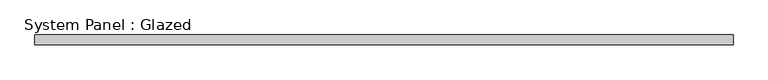
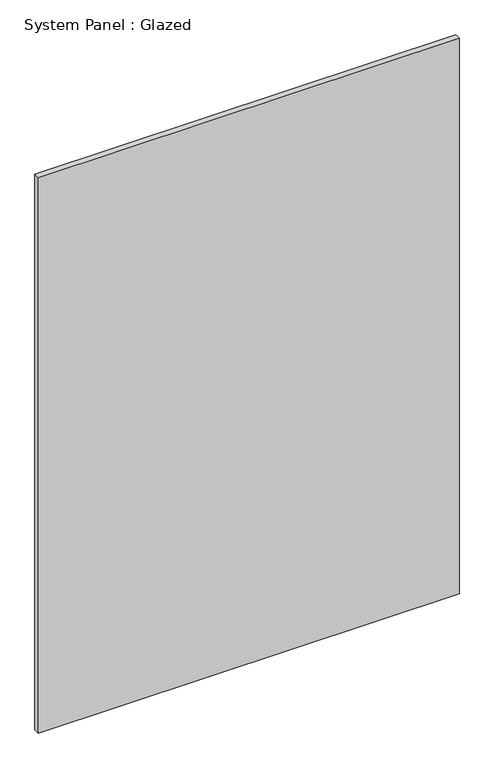
"""IFC4 building model written with IfcOpenShell, lengths in millimetres: plate geometry, System Panel : Glazed."""

import ifcopenshell
import ifcopenshell.guid

model = None  # the IFC model being written
_history = None  # IfcOwnerHistory: only IFC2X3 demands one
_inside = {}  # id of a spatial element -> (the spatial element, [elements in it])
_under = {}  # id of a project, library or spatial element -> (it, [spatial elements below it])
_declared = {}  # id of a project -> (the project, [libraries it declares])
_typed = {}  # id of a type object -> (the type object, [elements of that type])
_made_of = {}  # id of a material, layer set ... -> (it, [elements and type objects made of it])


def new_model(schema):
    """Start an empty IFC model of exactly this schema.

    Asked for "IFC4X3", IfcOpenShell would pick the latest addendum, in which some entities
    have other attributes; the version numbers below select the first issue.
    IFC2X3 requires an IfcOwnerHistory on every rooted entity: one is made here for all.
    """
    global model, _history
    if schema == "IFC4X3":
        model = ifcopenshell.file(schema_version=(4, 3, 0, 0))
    else:
        model = ifcopenshell.file(schema=schema)
    _inside.clear()
    _under.clear()
    _declared.clear()
    _typed.clear()
    _made_of.clear()
    _history = None
    if model.schema == "IFC2X3":
        org = make("IfcOrganization", Name="unknown")
        user = make(
            "IfcPersonAndOrganization",
            ThePerson=make("IfcPerson", FamilyName="unknown"),
            TheOrganization=org,
        )
        app = make(
            "IfcApplication",
            ApplicationDeveloper=org,
            Version="unknown",
            ApplicationFullName="unknown",
            ApplicationIdentifier="unknown",
        )
        _history = make(
            "IfcOwnerHistory",
            OwningUser=user,
            OwningApplication=app,
            ChangeAction="ADDED",
            CreationDate=0,
        )
    return model


def make(cls, **values):
    """One entity of the class cls with the attributes given. An attribute that is None is left unset."""
    return model.create_entity(
        cls, **{name: value for name, value in values.items() if value is not None}
    )


def rooted(cls, **values):
    """An entity with a GlobalId (a new one), such as an element, a storey or a relation."""
    return make(cls, GlobalId=ifcopenshell.guid.new(), OwnerHistory=_history, **values)


def si_unit(unit_type, name, prefix=None):
    """IfcSIUnit, for example si_unit("LENGTHUNIT", "METRE", prefix="MILLI")."""
    return make("IfcSIUnit", UnitType=unit_type, Prefix=prefix, Name=name)


def assignment(units):
    """IfcUnitAssignment: the units of a project."""
    return None if units is None else make("IfcUnitAssignment", Units=units)


def point(xyz):
    """IfcCartesianPoint."""
    return None if xyz is None else make("IfcCartesianPoint", Coordinates=xyz)


def direction(xyz):
    """IfcDirection."""
    return None if xyz is None else make("IfcDirection", DirectionRatios=xyz)


def frame(location, z_axis=None, x_axis=None):
    """IfcAxis2Placement3D, a coordinate frame: its origin and axes. An axis left out is left unset."""
    return make(
        "IfcAxis2Placement3D",
        Location=point(location),
        Axis=direction(z_axis),
        RefDirection=direction(x_axis),
    )


def origin():
    """The frame at (0, 0, 0) with its axes left unset."""
    return frame((0.0, 0.0, 0.0))


def origin_with_axes():
    """The frame at (0, 0, 0) with the z axis (0, 0, 1) and the x axis (1, 0, 0) written out."""
    return frame((0.0, 0.0, 0.0), z_axis=(0.0, 0.0, 1.0), x_axis=(1.0, 0.0, 0.0))


def place(relative_to, where):
    """IfcLocalPlacement: puts the frame where relative to a parent placement (None: the world)."""
    return make(
        "IfcLocalPlacement", PlacementRelTo=relative_to, RelativePlacement=where
    )


def context(
    kind, dimensions, precision=None, world=None, true_north=None, identifier=None
):
    """IfcGeometricRepresentationContext, for example the 3D "Model" context."""
    return make(
        "IfcGeometricRepresentationContext",
        ContextIdentifier=identifier,
        ContextType=kind,
        CoordinateSpaceDimension=dimensions,
        Precision=precision,
        WorldCoordinateSystem=world,
        TrueNorth=true_north,
    )


def project(units=None, contexts=None):
    """IfcProject with its units and contexts."""
    return rooted(
        "IfcProject",
        Name="project",
        RepresentationContexts=contexts,
        UnitsInContext=assignment(units),
    )


def spatial(cls, under=None, at=None, **own):
    """A site, building, storey or space (cls), placed at a placement, below another one or the project."""
    s = rooted(cls, ObjectPlacement=at, **own)
    if under is not None:
        _under.setdefault(under.id(), (under, []))[1].append(s)
    return s


def polyline(points):
    """IfcPolyline through the points."""
    return make("IfcPolyline", Points=[point(p) for p in points])


def outline(outer, holes=None, kind="AREA"):
    """IfcArbitraryClosedProfileDef: a profile drawn as a closed curve; with holes, ...WithVoids."""
    if holes is None:
        return make("IfcArbitraryClosedProfileDef", ProfileType=kind, OuterCurve=outer)
    return make(
        "IfcArbitraryProfileDefWithVoids",
        ProfileType=kind,
        OuterCurve=outer,
        InnerCurves=holes,
    )


def extrude(swept, where, along, depth):
    """IfcExtrudedAreaSolid: the profile swept, set in the frame where, extruded along a direction by depth."""
    return make(
        "IfcExtrudedAreaSolid",
        SweptArea=swept,
        Position=where,
        ExtrudedDirection=direction(along),
        Depth=depth,
    )


def shape(context_of_items, identifier, shape_type, items):
    """IfcShapeRepresentation: the items that make up one representation, for example the "Body"."""
    return make(
        "IfcShapeRepresentation",
        ContextOfItems=context_of_items,
        RepresentationIdentifier=identifier,
        RepresentationType=shape_type,
        Items=items,
    )


def source(mapping_origin, context_of_items, identifier, shape_type, items):
    """IfcRepresentationMap: a shape defined once, which mapped items show again and again."""
    return make(
        "IfcRepresentationMap",
        MappingOrigin=mapping_origin,
        MappedRepresentation=shape(context_of_items, identifier, shape_type, items),
    )


def transform(
    local_origin,
    x_axis=None,
    y_axis=None,
    z_axis=None,
    scale=None,
    scale2=None,
    scale3=None,
    uniform=True,
):
    """IfcCartesianTransformationOperator3D, or its non-uniform kind. x_axis, y_axis, z_axis: its Axis1, 2, 3."""
    if uniform:
        return make(
            "IfcCartesianTransformationOperator3D",
            Axis1=direction(x_axis),
            Axis2=direction(y_axis),
            LocalOrigin=point(local_origin),
            Scale=scale,
            Axis3=direction(z_axis),
        )
    return make(
        "IfcCartesianTransformationOperator3DnonUniform",
        Axis1=direction(x_axis),
        Axis2=direction(y_axis),
        LocalOrigin=point(local_origin),
        Scale=scale,
        Axis3=direction(z_axis),
        Scale2=scale2,
        Scale3=scale3,
    )


def mapped(mapping_source, mapping_target):
    """IfcMappedItem: shows the shape of a source again, moved by a transform."""
    return make(
        "IfcMappedItem", MappingSource=mapping_source, MappingTarget=mapping_target
    )


def made_of(thing, what):
    """Note that an element or type object is made of a material, layer set ...; save() writes the relation."""
    if what is not None:
        _made_of.setdefault(what.id(), (what, []))[1].append(thing)
    return thing


def element(
    cls,
    number,
    at=None,
    inside=None,
    cuts=None,
    type_object=None,
    material=None,
    context=None,
    identifier="Body",
    shape_type=None,
    held_by="IfcProductDefinitionShape",
    body=None,
    shapes=None,
    **own,
):
    """One element of the class cls, such as IfcWall. Its Tag is "e" and its number.

    at: its placement. inside: the storey or other place that contains it. cuts: it is an
    opening in that element (IfcRelVoidsElement). A single representation is given by context,
    identifier, shape_type and body (its items); several are given by shapes. held_by: the class
    of the entity that holds the representations. save() writes the other relations.
    """
    e = rooted(cls, Tag="e%d" % number, ObjectPlacement=at, **own)
    if body is not None:
        shapes = [shape(context, identifier, shape_type, body)]
    if shapes is not None:
        e.Representation = make(held_by, Representations=shapes)
    if inside is not None:
        _inside.setdefault(inside.id(), (inside, []))[1].append(e)
    if cuts is not None:
        rooted(
            "IfcRelVoidsElement", RelatingBuildingElement=cuts, RelatedOpeningElement=e
        )
    if type_object is not None:
        _typed.setdefault(type_object.id(), (type_object, []))[1].append(e)
    return made_of(e, material)


def aggregate(whole, parts):
    """IfcRelAggregates: a whole, such as a stair, and the parts it consists of."""
    return rooted("IfcRelAggregates", RelatingObject=whole, RelatedObjects=parts)


def save(model, path):
    """Write the relations noted so far, then the file.

    IfcRelAggregates (storeys below a building ...), IfcRelContainedInSpatialStructure (elements
    in a storey), IfcRelDefinesByType, IfcRelAssociatesMaterial and IfcRelDeclares: one each for
    every whole, place, type object, material and project.
    """
    for whole, parts in _under.values():
        aggregate(whole, parts)
    for where, things in _inside.values():
        rooted(
            "IfcRelContainedInSpatialStructure",
            RelatedElements=things,
            RelatingStructure=where,
        )
    for kind, things in _typed.values():
        rooted("IfcRelDefinesByType", RelatedObjects=things, RelatingType=kind)
    for what, things in _made_of.values():
        rooted("IfcRelAssociatesMaterial", RelatedObjects=things, RelatingMaterial=what)
    for by, libraries in _declared.values():
        rooted("IfcRelDeclares", RelatingContext=by, RelatedDefinitions=libraries)
    model.write(path)


def system_panel_glazed_ccadeef2(model_context):
    return source(origin(), model_context, "Body", "SweptSolid", [
        extrude(outline(polyline([(877.5, -49.5), (-877.5, -49.5), (-877.5, -24.5), (877.5, -24.5), (877.5, -49.5)])), origin_with_axes(), (0.0, 0.0, 1.0), 2450.0),
    ])


if __name__ == "__main__":
    model = new_model("IFC4")
    model_context = context("Model", 3, world=origin())
    ifc_project = project(units=[si_unit("LENGTHUNIT", "METRE", prefix="MILLI")], contexts=[model_context])
    site = spatial("IfcSite", under=ifc_project)
    building = spatial("IfcBuilding", under=site)
    placement = place(None, origin())
    system_panel_glazed_shape = system_panel_glazed_ccadeef2(model_context)
    element("IfcPlate", 1, ObjectType="System Panel : Glazed", at=placement, inside=building, context=model_context, shape_type="MappedRepresentation", body=[
        mapped(system_panel_glazed_shape, transform((0.0, 0.0, 0.0), x_axis=(1.0, 0.0, 0.0), y_axis=(0.0, 1.0, 0.0), z_axis=(0.0, 0.0, 1.0))),
    ])
    save(model, "model.ifc")

# Revit data of these elements
# Type "System Panel : Glazed"
#   Keynote = "H11"
#   Construction Type Id = "GSP4R"
#   Analytic Construction = "1/8 in Pilkington single glazing"
#   Visual Light Transmittance = 0.9
#   Solar Heat Gain Coefficient = 0.86
#   Heat Transfer Coefficient (U) = 6.7069 W/(m²·K)
# Element 1 (IfcPlate, "System Panel : Glazed")
#   Materials on its faces: "Glass"
# Materials
#   "Glass": class "Glass", colour RGB 0 128 192, transparency 0.9, Description = "Soda Lime Glass", Cost = 0
